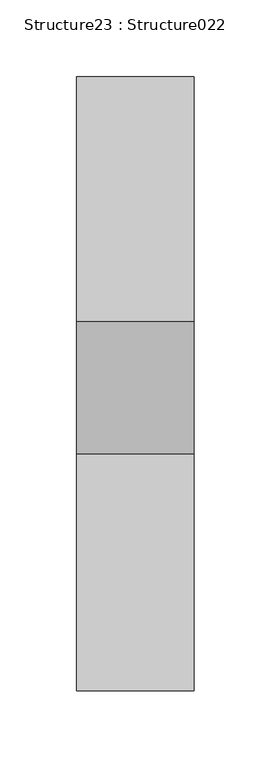
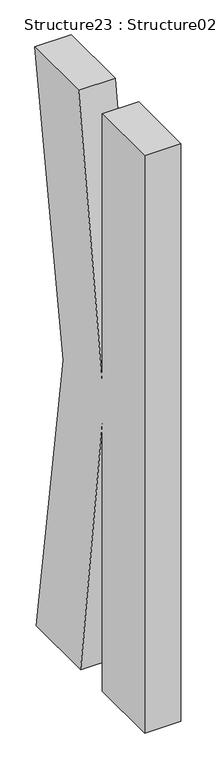
"""IFC4 building model written with IfcOpenShell, lengths in millimetres: proxy geometry, Structure23 : Structure022."""

from ifc_helpers import new_model, si_unit, frame, origin, place, context, project, spatial, polyline, outline, extrude, source, transform, mapped, element, save


def structure23_structure022_c342959d(model_context):
    return source(origin(), model_context, "Body", "SweptSolid", [
        extrude(outline(polyline([(654.7606267, 0.0), (630.9253781, -159.1897613), (33.1452881, -149.2088698), (619.2794757, -236.9698787), (596.5228349, -388.9558844), (-669.7923378, -199.3523782), (-647.035697, -47.3663725), (-59.1043408, -135.3964687), (-634.3060435, 37.6518519), (-610.7408859, 195.0377419), (0.0, 0.0), (654.7606267, 0.0)])), frame((-35624.0862846, 276371.2885381, 5127.2087404), z_axis=(1.0, 0.0, 1.354250045437766e-12), x_axis=(1.3421085009500405e-12, 0.148077875868084, -0.9889757037856878)), (0.0, 0.0, 1.0), 76.2),
    ])


if __name__ == "__main__":
    model = new_model("IFC4")
    model_context = context("Model", 3, world=origin())
    ifc_project = project(units=[si_unit("LENGTHUNIT", "METRE", prefix="MILLI")], contexts=[model_context])
    site = spatial("IfcSite", under=ifc_project)
    building = spatial("IfcBuilding", under=site)
    placement = place(None, origin())
    structure23_structure022_shape = structure23_structure022_c342959d(model_context)
    element("IfcBuildingElementProxy", 1, Name="Structure23 : Structure022", ObjectType="Structure23 : Structure022", at=placement, inside=building, context=model_context, shape_type="MappedRepresentation", body=[
        mapped(structure23_structure022_shape, transform((0.0, 0.0, 0.0), x_axis=(1.0, 0.0, 0.0), y_axis=(0.0, 1.0, 0.0), z_axis=(0.0, 0.0, 1.0))),
    ])
    save(model, "model.ifc")

# Revit data of these elements
# Type "Structure23 : Structure022"
#   NameOverride = "Structure022"
# Element 1 (IfcBuildingElementProxy, "Structure23 : Structure022")
#   Materials on its faces: "BRUSHED ALUMINUM LETTERING"
# Materials
#   "BRUSHED ALUMINUM LETTERING": class "Unassigned", colour RGB 169 181 186, transparency 0, Cost = 0
